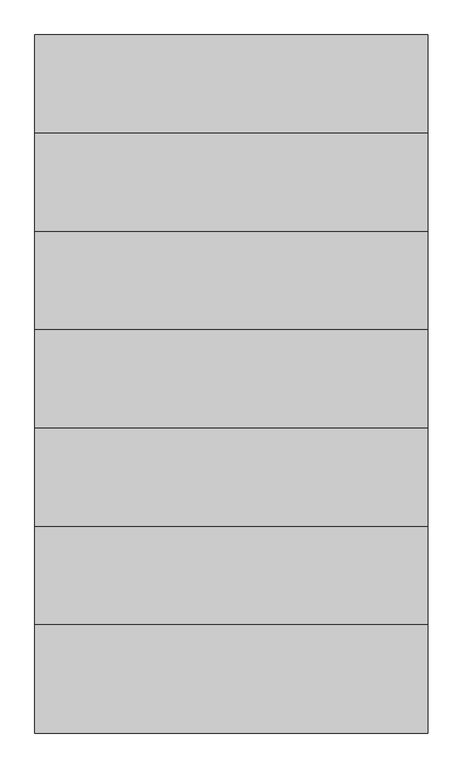
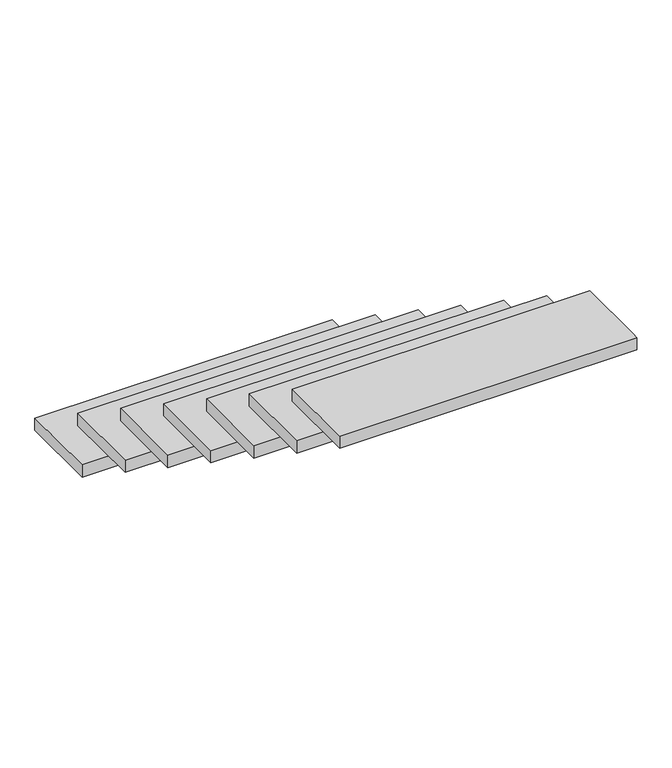
"""IFC4 building model written with IfcOpenShell, lengths in millimetres: stair flight geometry."""

from ifc_helpers import new_model, si_unit, frame, origin, place, context, project, spatial, polyline, outline, extrude, source, transform, mapped, element, save


def stair_flight_370392ba(model_context):
    return source(origin(), model_context, "Body", "SweptSolid", [
        extrude(outline(polyline([(-54750.7723171, 249784.749125), (-55766.7723171, 249784.749125), (-55766.7723171, 250064.149125), (-54750.7723171, 250064.149125), (-54750.7723171, 249784.749125)])), frame((0.0, 0.0, 127.0), z_axis=(0.0, 0.0, 1.0), x_axis=(1.0, 0.0, 0.0)), (0.0, 0.0, 1.0), 44.45),
        extrude(outline(polyline([(-54750.7723171, 249530.749125), (-55766.7723171, 249530.749125), (-55766.7723171, 249810.149125), (-54750.7723171, 249810.149125), (-54750.7723171, 249530.749125)])), frame((0.0, 0.0, 298.45), z_axis=(0.0, 0.0, 1.0), x_axis=(1.0, 0.0, 0.0)), (0.0, 0.0, 1.0), 44.45),
        extrude(outline(polyline([(-54750.7723171, 249276.749125), (-55766.7723171, 249276.749125), (-55766.7723171, 249556.149125), (-54750.7723171, 249556.149125), (-54750.7723171, 249276.749125)])), frame((0.0, 0.0, 469.9), z_axis=(0.0, 0.0, 1.0), x_axis=(1.0, 0.0, 0.0)), (0.0, 0.0, 1.0), 44.45),
        extrude(outline(polyline([(-54750.7723171, 249022.749125), (-55766.7723171, 249022.749125), (-55766.7723171, 249302.149125), (-54750.7723171, 249302.149125), (-54750.7723171, 249022.749125)])), frame((0.0, 0.0, 641.35), z_axis=(0.0, 0.0, 1.0), x_axis=(1.0, 0.0, 0.0)), (0.0, 0.0, 1.0), 44.45),
        extrude(outline(polyline([(-54750.7723171, 248768.749125), (-55766.7723171, 248768.749125), (-55766.7723171, 249048.149125), (-54750.7723171, 249048.149125), (-54750.7723171, 248768.749125)])), frame((0.0, 0.0, 812.8), z_axis=(0.0, 0.0, 1.0), x_axis=(1.0, 0.0, 0.0)), (0.0, 0.0, 1.0), 44.45),
        extrude(outline(polyline([(-54750.7723171, 248514.749125), (-55766.7723171, 248514.749125), (-55766.7723171, 248794.149125), (-54750.7723171, 248794.149125), (-54750.7723171, 248514.749125)])), frame((0.0, 0.0, 984.25), z_axis=(0.0, 0.0, 1.0), x_axis=(1.0, 0.0, 0.0)), (0.0, 0.0, 1.0), 44.45),
        extrude(outline(polyline([(-54750.7723171, 248260.749125), (-55766.7723171, 248260.749125), (-55766.7723171, 248540.149125), (-54750.7723171, 248540.149125), (-54750.7723171, 248286.149125), (-54750.7723171, 248260.749125)])), frame((0.0, 0.0, 1155.7), z_axis=(0.0, 0.0, 1.0), x_axis=(1.0, 0.0, 0.0)), (0.0, 0.0, 1.0), 44.45),
    ])


if __name__ == "__main__":
    model = new_model("IFC4")
    model_context = context("Model", 3, world=origin())
    ifc_project = project(units=[si_unit("LENGTHUNIT", "METRE", prefix="MILLI")], contexts=[model_context])
    site = spatial("IfcSite", under=ifc_project)
    building = spatial("IfcBuilding", under=site)
    placement = place(None, origin())
    stair_flight_shape = stair_flight_370392ba(model_context)
    element("IfcStairFlight", 1, at=placement, inside=building, context=model_context, shape_type="MappedRepresentation", body=[
        mapped(stair_flight_shape, transform((0.0, 0.0, 0.0), x_axis=(1.0, 0.0, 0.0), y_axis=(0.0, 1.0, 0.0), z_axis=(0.0, 0.0, 1.0))),
    ])
    save(model, "model.ifc")

# Revit data of these elements
# Element 1 (IfcStairFlight)
#   Materials on its faces: "Wood - Flooring"
# Materials
#   "Wood - Flooring": class "Unassigned", colour RGB 216 169 114, transparency 0
